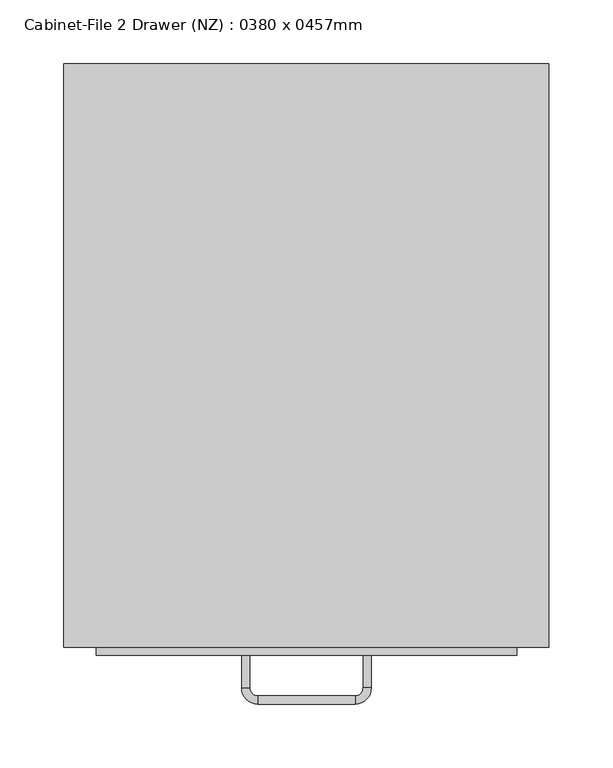
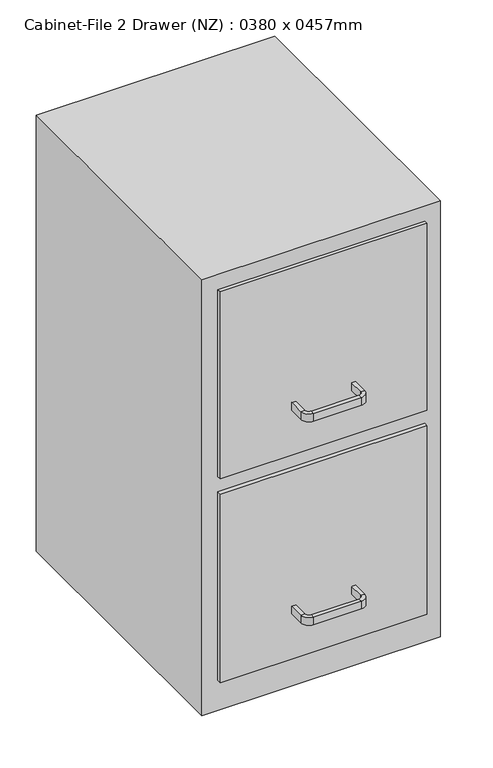
"""IFC4 building model written with IfcOpenShell, lengths in millimetres: furniture geometry, Cabinet-File 2 Drawer (NZ) : 0380 x 0457mm."""

from ifc_helpers import new_model, si_unit, frame, origin, origin_with_axes, place, context, project, spatial, polyline, circle_curve, outline, extrude, source, transform, mapped, element, save
from ifc_brep_helpers import plane_surface, cylinder_surface, revolved_surface, advanced_brep


def cabinet_file_2_drawer_nz_0380_x_0457mm_9eec7cff(model_context):
    return source(origin(), model_context, "Body", "SolidModel", [
        extrude(outline(polyline([(36.703553, -376.9843001), (-292.496447, -376.9843001), (-292.496447, -370.6343001), (36.703553, -370.6343001), (36.703553, -376.9843001)])), frame((0.0, 0.0, 393.7), z_axis=(0.0, 0.0, 1.0), x_axis=(1.0, 0.0, 0.0)), (0.0, 0.0, 1.0), 314.9),
        extrude(outline(polyline([(36.703553, -376.9843001), (-292.496447, -376.9843001), (-292.496447, -370.6343001), (36.703553, -370.6343001), (36.703553, -376.9843001)])), frame((0.0, 0.0, 50.8), z_axis=(0.0, 0.0, 1.0), x_axis=(1.0, 0.0, 0.0)), (0.0, 0.0, 1.0), 317.5),
        advanced_brep(
        [(-172.346447, -376.9843001, 127.0), (-178.696447, -376.9843001, 127.0), (-178.696447, -376.9843001, 139.7), (-172.346447, -376.9843001, 139.7), (-172.346447, -402.3843001, 127.0), (-178.696447, -402.3843001, 127.0), (-178.696447, -402.3843001, 139.7), (-172.346447, -402.3843001, 139.7), (-165.996447, -415.0843001, 127.0), (-165.996447, -408.7343001, 127.0), (-165.996447, -415.0843001, 139.7), (-165.996447, -408.7343001, 139.7), (-89.796447, -408.7343001, 127.0), (-89.796447, -415.0843001, 127.0), (-89.796447, -415.0843001, 139.7), (-89.796447, -408.7343001, 139.7), (-77.096447, -402.3843001, 127.0), (-83.446447, -402.3843001, 127.0), (-77.096447, -402.3843001, 139.7), (-83.446447, -402.3843001, 139.7), (-83.446447, -376.9843001, 127.0), (-83.446447, -376.9843001, 139.7), (-77.096447, -376.9843001, 139.7), (-77.096447, -376.9843001, 127.0)],
        [
            (0, 1),
            (1, 2),
            (2, 3),
            (3, 0),
            (0, 4),
            (4, 5),
            (5, 1),
            (5, 6),
            (6, 2),
            (6, 7),
            (7, 3),
            (7, 4),
            (8, 5, circle_curve(frame((-165.996447, -402.3843001, 127.0), z_axis=(0.0, 0.0, -1.0), x_axis=(-1.0, 0.0, 0.0)), 12.7)),
            (4, 9, circle_curve(frame((-165.996447, -402.3843001, 127.0), z_axis=(0.0, 0.0, 1.0), x_axis=(-1.0, 0.0, 0.0)), 6.35)),
            (9, 8),
            (10, 6, circle_curve(frame((-165.996447, -402.3843001, 139.7), z_axis=(0.0, 0.0, -1.0), x_axis=(-1.0, 0.0, 0.0)), 12.7)),
            (8, 10),
            (11, 7, circle_curve(frame((-165.996447, -402.3843001, 139.7), z_axis=(0.0, 0.0, -1.0), x_axis=(-1.0, 0.0, 0.0)), 6.35)),
            (10, 11),
            (11, 9),
            (9, 12),
            (12, 13),
            (13, 8),
            (13, 14),
            (14, 10),
            (14, 15),
            (15, 11),
            (15, 12),
            (16, 13, circle_curve(frame((-89.796447, -402.3843001, 127.0), z_axis=(0.0, 0.0, -1.0), x_axis=(0.0, -1.0, 0.0)), 12.7)),
            (12, 17, circle_curve(frame((-89.796447, -402.3843001, 127.0), z_axis=(0.0, 0.0, 1.0), x_axis=(0.0, -1.0, 0.0)), 6.35)),
            (17, 16),
            (18, 14, circle_curve(frame((-89.796447, -402.3843001, 139.7), z_axis=(0.0, 0.0, -1.0), x_axis=(0.0, -1.0, 0.0)), 12.7)),
            (16, 18),
            (19, 15, circle_curve(frame((-89.796447, -402.3843001, 139.7), z_axis=(0.0, 0.0, -1.0), x_axis=(0.0, -1.0, 0.0)), 6.35)),
            (18, 19),
            (19, 17),
            (20, 21),
            (21, 22),
            (22, 23),
            (23, 20),
            (17, 20),
            (23, 16),
            (22, 18),
            (21, 19),
        ],
        [
            plane_surface(frame((-661.3382215, -376.9843001, 0.0), z_axis=(0.0, 1.0, 0.0), x_axis=(0.0, 0.0, -1.0))),
            plane_surface(frame((-172.346447, -376.9843001, 127.0), z_axis=(0.0, 0.0, -1.0), x_axis=(0.0, -1.0, 0.0))),
            plane_surface(frame((-178.696447, -376.9843001, 127.0), z_axis=(-1.0, 0.0, 0.0), x_axis=(0.0, -1.0, 0.0))),
            plane_surface(frame((-178.696447, -376.9843001, 139.7), z_axis=(0.0, 0.0, 1.0), x_axis=(0.0, -1.0, 0.0))),
            plane_surface(frame((-172.346447, -376.9843001, 139.7), z_axis=(1.0, 0.0, 0.0), x_axis=(0.0, -1.0, 0.0))),
            plane_surface(frame((-165.996447, -402.3843001, 127.0), z_axis=(0.0, 0.0, -1.0), x_axis=(-1.0, 0.0, 0.0))),
            cylinder_surface(frame((-165.996447, -402.3843001, 0.0), z_axis=(0.0, 0.0, 1.0), x_axis=(-1.0, 0.0, 0.0)), 12.7),
            plane_surface(frame((-165.996447, -402.3843001, 139.7), z_axis=(0.0, 0.0, 1.0), x_axis=(-1.0, 0.0, 0.0))),
            revolved_surface(polyline([(-172.34644699999998, -402.3843001, 139.7), (-172.34644699999998, -402.3843001, 127.0)]), (-165.996447, -402.3843001, 0.0), (0.0, 0.0, 1.0)),
            plane_surface(frame((-165.996447, -408.7343001, 127.0), z_axis=(0.0, 0.0, -1.0), x_axis=(1.0, 0.0, 0.0))),
            plane_surface(frame((-165.996447, -415.0843001, 127.0), z_axis=(0.0, -1.0, 0.0), x_axis=(1.0, 0.0, 0.0))),
            plane_surface(frame((-165.996447, -415.0843001, 139.7), z_axis=(0.0, 0.0, 1.0), x_axis=(1.0, 0.0, 0.0))),
            plane_surface(frame((-165.996447, -408.7343001, 139.7), z_axis=(0.0, 1.0, 0.0), x_axis=(1.0, 0.0, 0.0))),
            plane_surface(frame((-89.796447, -402.3843001, 127.0), z_axis=(0.0, 0.0, -1.0), x_axis=(0.0, -1.0, 0.0))),
            cylinder_surface(frame((-89.796447, -402.3843001, 0.0), z_axis=(0.0, 0.0, 1.0), x_axis=(0.0, -1.0, 0.0)), 12.7),
            plane_surface(frame((-89.796447, -402.3843001, 139.7), z_axis=(0.0, 0.0, 1.0), x_axis=(0.0, -1.0, 0.0))),
            revolved_surface(polyline([(-89.796447, -408.73430010000004, 139.7), (-89.796447, -408.73430010000004, 127.0)]), (-89.796447, -402.3843001, 0.0), (0.0, 0.0, 1.0)),
            plane_surface(frame((-559.7382215, -376.9843001, 0.0), z_axis=(0.0, 1.0, 0.0), x_axis=(0.0, 0.0, 1.0))),
            plane_surface(frame((-83.446447, -402.3843001, 127.0), z_axis=(0.0, 0.0, -1.0), x_axis=(0.0, 1.0, 0.0))),
            plane_surface(frame((-77.096447, -402.3843001, 127.0), z_axis=(1.0, 0.0, 0.0), x_axis=(0.0, 1.0, 0.0))),
            plane_surface(frame((-77.096447, -402.3843001, 139.7), z_axis=(0.0, 0.0, 1.0), x_axis=(0.0, 1.0, 0.0))),
            plane_surface(frame((-83.446447, -402.3843001, 139.7), z_axis=(-1.0, 0.0, 0.0), x_axis=(0.0, 1.0, 0.0))),
        ],
        [
            (0, [[1, 2, 3, 4]]),
            (1, [[-1, 5, 6, 7]]),
            (2, [[-2, -7, 8, 9]]),
            (3, [[-3, -9, 10, 11]]),
            (4, [[-4, -11, 12, -5]]),
            (5, [[13, -6, 14, 15]]),
            (6, [[16, -8, -13, 17]]),
            (7, [[18, -10, -16, 19]]),
            (8, [[-14, -12, -18, 20]]),
            (9, [[-15, 21, 22, 23]]),
            (10, [[-17, -23, 24, 25]]),
            (11, [[-19, -25, 26, 27]]),
            (12, [[-20, -27, 28, -21]]),
            (13, [[29, -22, 30, 31]]),
            (14, [[32, -24, -29, 33]]),
            (15, [[34, -26, -32, 35]]),
            (16, [[-30, -28, -34, 36]]),
            (17, [[37, 38, 39, 40]]),
            (18, [[-31, 41, -40, 42]]),
            (19, [[-33, -42, -39, 43]]),
            (20, [[-35, -43, -38, 44]]),
            (21, [[-36, -44, -37, -41]]),
        ],
    ),
        advanced_brep(
        [(-172.346447, -376.9843001, 469.9), (-178.696447, -376.9843001, 469.9), (-178.696447, -376.9843001, 482.6), (-172.346447, -376.9843001, 482.6), (-172.346447, -402.3843001, 469.9), (-178.696447, -402.3843001, 469.9), (-178.696447, -402.3843001, 482.6), (-172.346447, -402.3843001, 482.6), (-165.996447, -415.0843001, 469.9), (-165.996447, -408.7343001, 469.9), (-165.996447, -415.0843001, 482.6), (-165.996447, -408.7343001, 482.6), (-89.796447, -408.7343001, 469.9), (-89.796447, -415.0843001, 469.9), (-89.796447, -415.0843001, 482.6), (-89.796447, -408.7343001, 482.6), (-77.096447, -402.3843001, 469.9), (-83.446447, -402.3843001, 469.9), (-77.096447, -402.3843001, 482.6), (-83.446447, -402.3843001, 482.6), (-83.446447, -376.9843001, 469.9), (-83.446447, -376.9843001, 482.6), (-77.096447, -376.9843001, 482.6), (-77.096447, -376.9843001, 469.9)],
        [
            (0, 1),
            (1, 2),
            (2, 3),
            (3, 0),
            (0, 4),
            (4, 5),
            (5, 1),
            (5, 6),
            (6, 2),
            (6, 7),
            (7, 3),
            (7, 4),
            (8, 5, circle_curve(frame((-165.996447, -402.3843001, 469.9), z_axis=(0.0, 0.0, -1.0), x_axis=(-1.0, 0.0, 0.0)), 12.7)),
            (4, 9, circle_curve(frame((-165.996447, -402.3843001, 469.9), z_axis=(0.0, 0.0, 1.0), x_axis=(-1.0, 0.0, 0.0)), 6.35)),
            (9, 8),
            (10, 6, circle_curve(frame((-165.996447, -402.3843001, 482.6), z_axis=(0.0, 0.0, -1.0), x_axis=(-1.0, 0.0, 0.0)), 12.7)),
            (8, 10),
            (11, 7, circle_curve(frame((-165.996447, -402.3843001, 482.6), z_axis=(0.0, 0.0, -1.0), x_axis=(-1.0, 0.0, 0.0)), 6.35)),
            (10, 11),
            (11, 9),
            (9, 12),
            (12, 13),
            (13, 8),
            (13, 14),
            (14, 10),
            (14, 15),
            (15, 11),
            (15, 12),
            (16, 13, circle_curve(frame((-89.796447, -402.3843001, 469.9), z_axis=(0.0, 0.0, -1.0), x_axis=(0.0, -1.0, 0.0)), 12.7)),
            (12, 17, circle_curve(frame((-89.796447, -402.3843001, 469.9), z_axis=(0.0, 0.0, 1.0), x_axis=(0.0, -1.0, 0.0)), 6.35)),
            (17, 16),
            (18, 14, circle_curve(frame((-89.796447, -402.3843001, 482.6), z_axis=(0.0, 0.0, -1.0), x_axis=(0.0, -1.0, 0.0)), 12.7)),
            (16, 18),
            (19, 15, circle_curve(frame((-89.796447, -402.3843001, 482.6), z_axis=(0.0, 0.0, -1.0), x_axis=(0.0, -1.0, 0.0)), 6.35)),
            (18, 19),
            (19, 17),
            (20, 21),
            (21, 22),
            (22, 23),
            (23, 20),
            (17, 20),
            (23, 16),
            (22, 18),
            (21, 19),
        ],
        [
            plane_surface(frame((-661.3382215, -376.9843001, 0.0), z_axis=(0.0, 1.0, 0.0), x_axis=(0.0, 0.0, -1.0))),
            plane_surface(frame((-172.346447, -376.9843001, 469.9), z_axis=(0.0, 0.0, -1.0), x_axis=(0.0, -1.0, 0.0))),
            plane_surface(frame((-178.696447, -376.9843001, 469.9), z_axis=(-1.0, 0.0, 0.0), x_axis=(0.0, -1.0, 0.0))),
            plane_surface(frame((-178.696447, -376.9843001, 482.6), z_axis=(0.0, 0.0, 1.0), x_axis=(0.0, -1.0, 0.0))),
            plane_surface(frame((-172.346447, -376.9843001, 482.6), z_axis=(1.0, 0.0, 0.0), x_axis=(0.0, -1.0, 0.0))),
            plane_surface(frame((-165.996447, -402.3843001, 469.9), z_axis=(0.0, 0.0, -1.0), x_axis=(-1.0, 0.0, 0.0))),
            cylinder_surface(frame((-165.996447, -402.3843001, 0.0), z_axis=(0.0, 0.0, 1.0), x_axis=(-1.0, 0.0, 0.0)), 12.7),
            plane_surface(frame((-165.996447, -402.3843001, 482.6), z_axis=(0.0, 0.0, 1.0), x_axis=(-1.0, 0.0, 0.0))),
            revolved_surface(polyline([(-172.34644699999998, -402.3843001, 482.6), (-172.34644699999998, -402.3843001, 469.9)]), (-165.996447, -402.3843001, 0.0), (0.0, 0.0, 1.0)),
            plane_surface(frame((-165.996447, -408.7343001, 469.9), z_axis=(0.0, 0.0, -1.0), x_axis=(1.0, 0.0, 0.0))),
            plane_surface(frame((-165.996447, -415.0843001, 469.9), z_axis=(0.0, -1.0, 0.0), x_axis=(1.0, 0.0, 0.0))),
            plane_surface(frame((-165.996447, -415.0843001, 482.6), z_axis=(0.0, 0.0, 1.0), x_axis=(1.0, 0.0, 0.0))),
            plane_surface(frame((-165.996447, -408.7343001, 482.6), z_axis=(0.0, 1.0, 0.0), x_axis=(1.0, 0.0, 0.0))),
            plane_surface(frame((-89.796447, -402.3843001, 469.9), z_axis=(0.0, 0.0, -1.0), x_axis=(0.0, -1.0, 0.0))),
            cylinder_surface(frame((-89.796447, -402.3843001, 0.0), z_axis=(0.0, 0.0, 1.0), x_axis=(0.0, -1.0, 0.0)), 12.7),
            plane_surface(frame((-89.796447, -402.3843001, 482.6), z_axis=(0.0, 0.0, 1.0), x_axis=(0.0, -1.0, 0.0))),
            revolved_surface(polyline([(-89.796447, -408.73430010000004, 482.6), (-89.796447, -408.73430010000004, 469.9)]), (-89.796447, -402.3843001, 0.0), (0.0, 0.0, 1.0)),
            plane_surface(frame((-559.7382215, -376.9843001, 0.0), z_axis=(0.0, 1.0, 0.0), x_axis=(0.0, 0.0, 1.0))),
            plane_surface(frame((-83.446447, -402.3843001, 469.9), z_axis=(0.0, 0.0, -1.0), x_axis=(0.0, 1.0, 0.0))),
            plane_surface(frame((-77.096447, -402.3843001, 469.9), z_axis=(1.0, 0.0, 0.0), x_axis=(0.0, 1.0, 0.0))),
            plane_surface(frame((-77.096447, -402.3843001, 482.6), z_axis=(0.0, 0.0, 1.0), x_axis=(0.0, 1.0, 0.0))),
            plane_surface(frame((-83.446447, -402.3843001, 482.6), z_axis=(-1.0, 0.0, 0.0), x_axis=(0.0, 1.0, 0.0))),
        ],
        [
            (0, [[1, 2, 3, 4]]),
            (1, [[-1, 5, 6, 7]]),
            (2, [[-2, -7, 8, 9]]),
            (3, [[-3, -9, 10, 11]]),
            (4, [[-4, -11, 12, -5]]),
            (5, [[13, -6, 14, 15]]),
            (6, [[16, -8, -13, 17]]),
            (7, [[18, -10, -16, 19]]),
            (8, [[-14, -12, -18, 20]]),
            (9, [[-15, 21, 22, 23]]),
            (10, [[-17, -23, 24, 25]]),
            (11, [[-19, -25, 26, 27]]),
            (12, [[-20, -27, 28, -21]]),
            (13, [[29, -22, 30, 31]]),
            (14, [[32, -24, -29, 33]]),
            (15, [[34, -26, -32, 35]]),
            (16, [[-30, -28, -34, 36]]),
            (17, [[37, 38, 39, 40]]),
            (18, [[-31, 41, -40, 42]]),
            (19, [[-33, -42, -39, 43]]),
            (20, [[-35, -43, -38, 44]]),
            (21, [[-36, -44, -37, -41]]),
        ],
    ),
        extrude(outline(polyline([(62.103553, 86.3656999), (62.103553, -370.6343001), (-317.896447, -370.6343001), (-317.896447, 86.3656999), (62.103553, 86.3656999)])), origin_with_axes(), (0.0, 0.0, 1.0), 734.0),
    ])


if __name__ == "__main__":
    model = new_model("IFC4")
    model_context = context("Model", 3, world=origin())
    ifc_project = project(units=[si_unit("LENGTHUNIT", "METRE", prefix="MILLI")], contexts=[model_context])
    site = spatial("IfcSite", under=ifc_project)
    building = spatial("IfcBuilding", under=site)
    placement = place(None, origin())
    cabinet_file_2_drawer_nz_0380_x_0457mm_shape = cabinet_file_2_drawer_nz_0380_x_0457mm_9eec7cff(model_context)
    element("IfcFurniture", 1, ObjectType="Cabinet-File 2 Drawer (NZ) : 0380 x 0457mm", at=placement, inside=building, context=model_context, shape_type="MappedRepresentation", body=[
        mapped(cabinet_file_2_drawer_nz_0380_x_0457mm_shape, transform((0.0, 0.0, 0.0), x_axis=(1.0, 0.0, 0.0), y_axis=(0.0, 1.0, 0.0), z_axis=(0.0, 0.0, 1.0))),
    ])
    save(model, "model.ifc")

# Revit data of these elements
# Type "Cabinet-File 2 Drawer (NZ) : 0380 x 0457mm"
#   Depth = 457 mm
#   Height = 734 mm
#   Width = 380 mm
#   Cabinet Material = Metal - Paint Finish - Ivory, Glossy
#   Handle Material = Metal - Chrome
# Element 1 (IfcFurniture, "Cabinet-File 2 Drawer (NZ) : 0380 x 0457mm")
#   Materials on its faces: "Metal - Chrome", "Metal - Paint Finish - Ivory, Glossy"
# Materials
#   "Metal - Paint Finish - Ivory, Glossy": class "Paint", colour RGB 247 247 239, transparency 0
#   "Metal - Chrome": class "Metal", colour RGB 17 17 17, transparency 0
